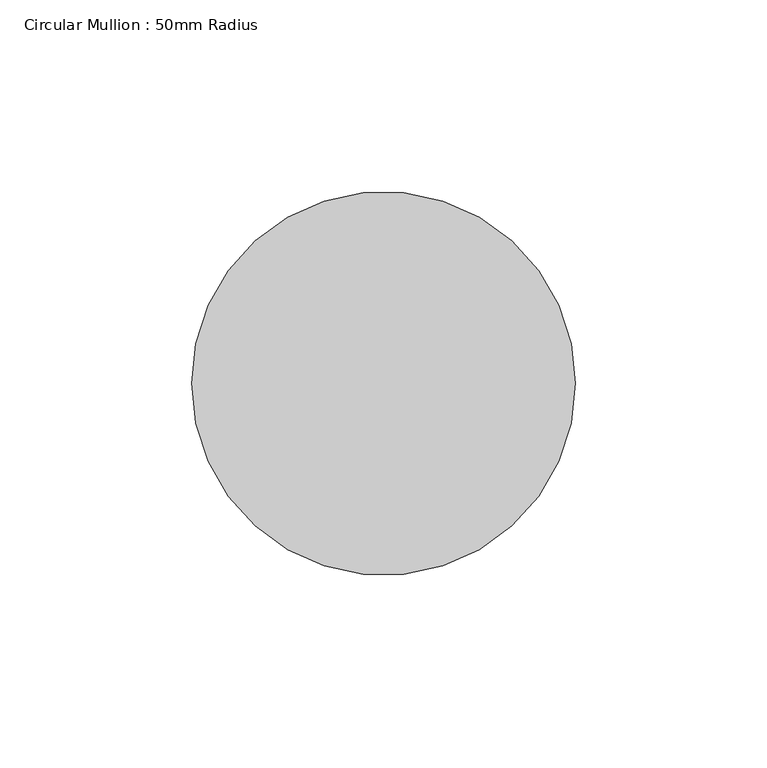
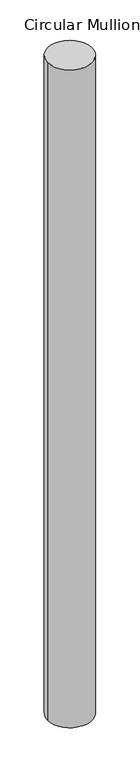
"""IFC4 building model written with IfcOpenShell, lengths in millimetres: member geometry, Circular Mullion : 50mm Radius."""

from ifc_helpers import new_model, si_unit, point, frame, origin, origin_2d, place, context, project, spatial, circle_curve, trimmed, segment, composite_curve, outline, extrude, source, transform, mapped, element, save


def circular_mullion_50mm_radius_db0fd72c(model_context):
    return source(origin(), model_context, "Body", "SweptSolid", [
        extrude(outline(composite_curve([segment(trimmed(circle_curve(origin_2d(), 50.0), [point((50.0, 0.0))], [point((-50.0, 0.0))], False, "CARTESIAN"), True, "CONTINUOUS"), segment(trimmed(circle_curve(origin_2d(), 50.0), [point((-50.0, 0.0))], [point((50.0, 0.0))], False, "CARTESIAN"), True, "CONTINUOUS")], self_intersect=False)), frame((0.0, 0.0, -1559.3436038), z_axis=(0.0, 0.0, 1.0), x_axis=(1.0, 0.0, 0.0)), (0.0, 0.0, 1.0), 1559.3436038),
    ])


if __name__ == "__main__":
    model = new_model("IFC4")
    model_context = context("Model", 3, world=origin())
    ifc_project = project(units=[si_unit("LENGTHUNIT", "METRE", prefix="MILLI")], contexts=[model_context])
    site = spatial("IfcSite", under=ifc_project)
    building = spatial("IfcBuilding", under=site)
    placement = place(None, origin())
    circular_mullion_50mm_radius_shape = circular_mullion_50mm_radius_db0fd72c(model_context)
    element("IfcMember", 1, ObjectType="Circular Mullion : 50mm Radius", at=placement, inside=building, context=model_context, shape_type="MappedRepresentation", body=[
        mapped(circular_mullion_50mm_radius_shape, transform((0.0, 0.0, 0.0), x_axis=(1.0, 0.0, 0.0), y_axis=(0.0, 1.0, 0.0), z_axis=(0.0, 0.0, 1.0))),
    ])
    save(model, "model.ifc")

# Revit data of these elements
# Type "Circular Mullion : 50mm Radius"
#   built-in parameter 1007350 = 0.164042 (stored number, unit not read)
# Element 1 (IfcMember, "Circular Mullion : 50mm Radius")
#   Materials on its faces: "Aluminium"
# Materials
#   "Aluminium": class "Metal", colour RGB 247 247 247, transparency 0, Description = "Aluminium 6061", Cost = 0
